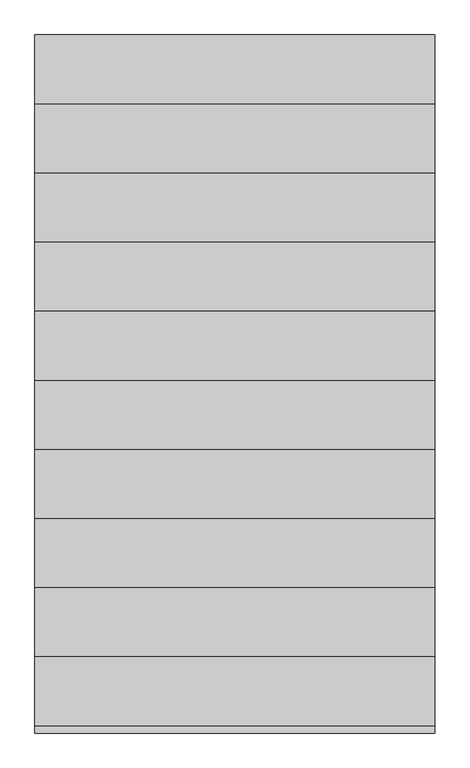
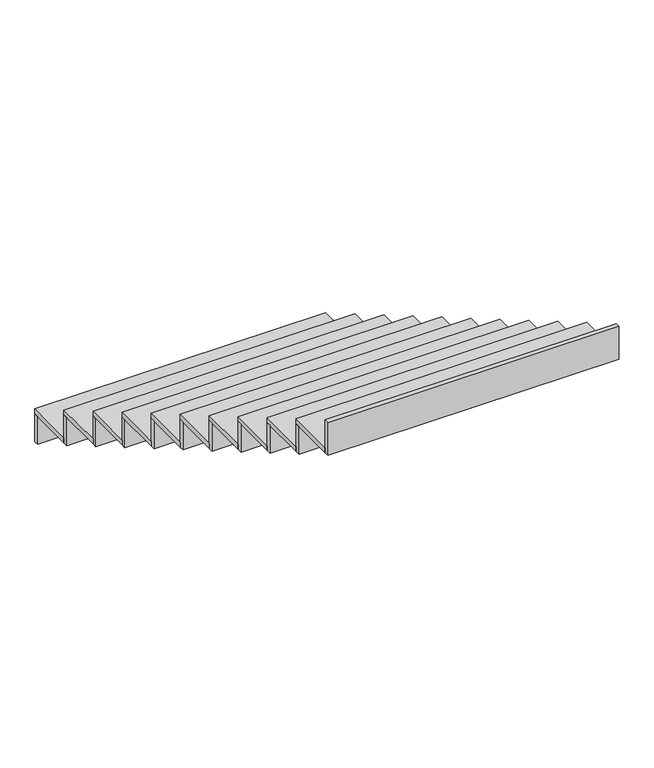
"""IFC4 building model written with IfcOpenShell, lengths in millimetres: stair flight geometry."""

from ifc_helpers import new_model, si_unit, frame, origin, place, context, project, spatial, polyline, outline, extrude, source, transform, mapped, element, save


def stair_flight_46729080(model_context):
    return source(origin(), model_context, "Body", "SweptSolid", [
        extrude(outline(polyline([(52915.0, -2680.0), (52915.0, -2650.0), (54650.0, -2650.0), (54650.0, -2680.0), (52915.0, -2680.0)])), frame((0.0, 0.0, 12145.0), z_axis=(0.0, 0.0, 1.0), x_axis=(1.0, 0.0, 0.0)), (0.0, 0.0, 1.0), 175.0),
        extrude(outline(polyline([(54650.0, -2950.0), (52915.0, -2950.0), (52915.0, -2650.0), (54650.0, -2650.0), (54650.0, -2950.0)])), frame((0.0, 0.0, 12320.0), z_axis=(0.0, 0.0, 1.0), x_axis=(1.0, 0.0, 0.0)), (0.0, 0.0, 1.0), 30.0),
        extrude(outline(polyline([(52915.0, -2980.0), (52915.0, -2950.0), (54650.0, -2950.0), (54650.0, -2980.0), (52915.0, -2980.0)])), frame((0.0, 0.0, 12320.0), z_axis=(0.0, 0.0, 1.0), x_axis=(1.0, 0.0, 0.0)), (0.0, 0.0, 1.0), 175.0),
        extrude(outline(polyline([(54650.0, -3250.0), (52915.0, -3250.0), (52915.0, -2950.0), (54650.0, -2950.0), (54650.0, -3250.0)])), frame((0.0, 0.0, 12495.0), z_axis=(0.0, 0.0, 1.0), x_axis=(1.0, 0.0, 0.0)), (0.0, 0.0, 1.0), 30.0),
        extrude(outline(polyline([(52915.0, -3280.0), (52915.0, -3250.0), (54650.0, -3250.0), (54650.0, -3280.0), (52915.0, -3280.0)])), frame((0.0, 0.0, 12495.0), z_axis=(0.0, 0.0, 1.0), x_axis=(1.0, 0.0, 0.0)), (0.0, 0.0, 1.0), 175.0),
        extrude(outline(polyline([(54650.0, -3550.0), (52915.0, -3550.0), (52915.0, -3250.0), (54650.0, -3250.0), (54650.0, -3550.0)])), frame((0.0, 0.0, 12670.0), z_axis=(0.0, 0.0, 1.0), x_axis=(1.0, 0.0, 0.0)), (0.0, 0.0, 1.0), 30.0),
        extrude(outline(polyline([(52915.0, -3580.0), (52915.0, -3550.0), (54650.0, -3550.0), (54650.0, -3580.0), (52915.0, -3580.0)])), frame((0.0, 0.0, 12670.0), z_axis=(0.0, 0.0, 1.0), x_axis=(1.0, 0.0, 0.0)), (0.0, 0.0, 1.0), 175.0),
        extrude(outline(polyline([(54650.0, -3850.0), (52915.0, -3850.0), (52915.0, -3550.0), (54650.0, -3550.0), (54650.0, -3850.0)])), frame((0.0, 0.0, 12845.0), z_axis=(0.0, 0.0, 1.0), x_axis=(1.0, 0.0, 0.0)), (0.0, 0.0, 1.0), 30.0),
        extrude(outline(polyline([(52915.0, -3880.0), (52915.0, -3850.0), (54650.0, -3850.0), (54650.0, -3880.0), (52915.0, -3880.0)])), frame((0.0, 0.0, 12845.0), z_axis=(0.0, 0.0, 1.0), x_axis=(1.0, 0.0, 0.0)), (0.0, 0.0, 1.0), 175.0),
        extrude(outline(polyline([(54650.0, -4150.0), (52915.0, -4150.0), (52915.0, -3850.0), (54650.0, -3850.0), (54650.0, -4150.0)])), frame((0.0, 0.0, 13020.0), z_axis=(0.0, 0.0, 1.0), x_axis=(1.0, 0.0, 0.0)), (0.0, 0.0, 1.0), 30.0),
        extrude(outline(polyline([(52915.0, -4180.0), (52915.0, -4150.0), (54650.0, -4150.0), (54650.0, -4180.0), (52915.0, -4180.0)])), frame((0.0, 0.0, 13020.0), z_axis=(0.0, 0.0, 1.0), x_axis=(1.0, 0.0, 0.0)), (0.0, 0.0, 1.0), 175.0),
        extrude(outline(polyline([(54650.0, -4450.0), (52915.0, -4450.0), (52915.0, -4150.0), (54650.0, -4150.0), (54650.0, -4450.0)])), frame((0.0, 0.0, 13195.0), z_axis=(0.0, 0.0, 1.0), x_axis=(1.0, 0.0, 0.0)), (0.0, 0.0, 1.0), 30.0),
        extrude(outline(polyline([(52915.0, -4480.0), (52915.0, -4450.0), (54650.0, -4450.0), (54650.0, -4480.0), (52915.0, -4480.0)])), frame((0.0, 0.0, 13195.0), z_axis=(0.0, 0.0, 1.0), x_axis=(1.0, 0.0, 0.0)), (0.0, 0.0, 1.0), 175.0),
        extrude(outline(polyline([(54650.0, -4750.0), (52915.0, -4750.0), (52915.0, -4450.0), (54650.0, -4450.0), (54650.0, -4750.0)])), frame((0.0, 0.0, 13370.0), z_axis=(0.0, 0.0, 1.0), x_axis=(1.0, 0.0, 0.0)), (0.0, 0.0, 1.0), 30.0),
        extrude(outline(polyline([(52915.0, -4780.0), (52915.0, -4750.0), (54650.0, -4750.0), (54650.0, -4780.0), (52915.0, -4780.0)])), frame((0.0, 0.0, 13370.0), z_axis=(0.0, 0.0, 1.0), x_axis=(1.0, 0.0, 0.0)), (0.0, 0.0, 1.0), 175.0),
        extrude(outline(polyline([(54650.0, -5050.0), (52915.0, -5050.0), (52915.0, -4750.0), (54650.0, -4750.0), (54650.0, -5050.0)])), frame((0.0, 0.0, 13545.0), z_axis=(0.0, 0.0, 1.0), x_axis=(1.0, 0.0, 0.0)), (0.0, 0.0, 1.0), 30.0),
        extrude(outline(polyline([(52915.0, -5080.0), (52915.0, -5050.0), (54650.0, -5050.0), (54650.0, -5080.0), (52915.0, -5080.0)])), frame((0.0, 0.0, 13545.0), z_axis=(0.0, 0.0, 1.0), x_axis=(1.0, 0.0, 0.0)), (0.0, 0.0, 1.0), 175.0),
        extrude(outline(polyline([(54650.0, -5350.0), (52915.0, -5350.0), (52915.0, -5050.0), (54650.0, -5050.0), (54650.0, -5350.0)])), frame((0.0, 0.0, 13720.0), z_axis=(0.0, 0.0, 1.0), x_axis=(1.0, 0.0, 0.0)), (0.0, 0.0, 1.0), 30.0),
        extrude(outline(polyline([(52915.0, -5380.0), (52915.0, -5350.0), (54650.0, -5350.0), (54650.0, -5380.0), (52915.0, -5380.0)])), frame((0.0, 0.0, 13720.0), z_axis=(0.0, 0.0, 1.0), x_axis=(1.0, 0.0, 0.0)), (0.0, 0.0, 1.0), 175.0),
        extrude(outline(polyline([(52915.0, -5680.0), (52915.0, -5650.0), (54650.0, -5650.0), (54650.0, -5680.0), (52915.0, -5680.0)])), frame((0.0, 0.0, 13895.0), z_axis=(0.0, 0.0, 1.0), x_axis=(1.0, 0.0, 0.0)), (0.0, 0.0, 1.0), 205.0),
        extrude(outline(polyline([(54650.0, -5650.0), (52915.0, -5650.0), (52915.0, -5350.0), (54650.0, -5350.0), (54650.0, -5650.0)])), frame((0.0, 0.0, 13895.0), z_axis=(0.0, 0.0, 1.0), x_axis=(1.0, 0.0, 0.0)), (0.0, 0.0, 1.0), 30.0),
    ])


if __name__ == "__main__":
    model = new_model("IFC4")
    model_context = context("Model", 3, world=origin())
    ifc_project = project(units=[si_unit("LENGTHUNIT", "METRE", prefix="MILLI")], contexts=[model_context])
    site = spatial("IfcSite", under=ifc_project)
    building = spatial("IfcBuilding", under=site)
    placement = place(None, origin())
    stair_flight_shape = stair_flight_46729080(model_context)
    element("IfcStairFlight", 1, at=placement, inside=building, context=model_context, shape_type="MappedRepresentation", body=[
        mapped(stair_flight_shape, transform((0.0, 0.0, 0.0), x_axis=(1.0, 0.0, 0.0), y_axis=(0.0, 1.0, 0.0), z_axis=(0.0, 0.0, 1.0))),
    ])
    save(model, "model.ifc")

# Revit data of these elements
# Element 1 (IfcStairFlight)
#   Materials on its faces: "00_Finish_Deco Tile"
# Materials
#   "00_Finish_Deco Tile": class "Finish", colour RGB 245 245 245, transparency 0, Description = "Ceramic Tile", Cost = 0
